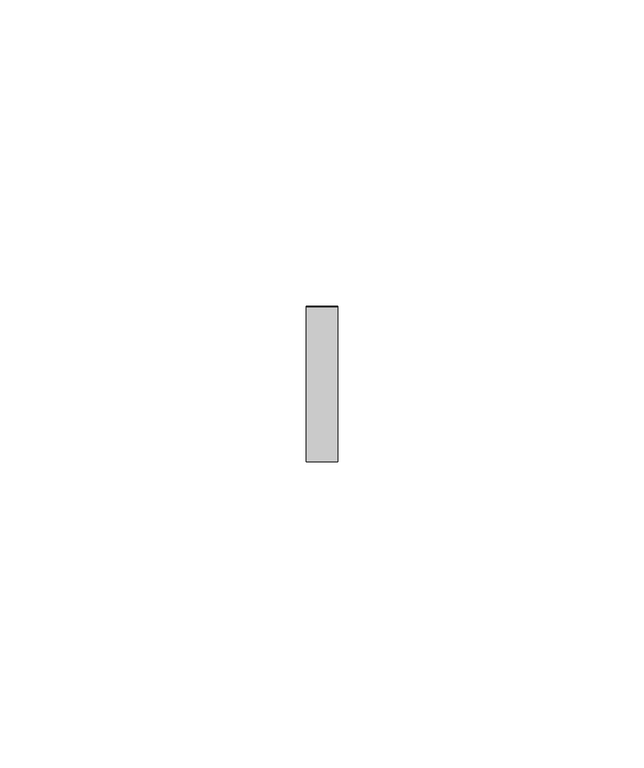
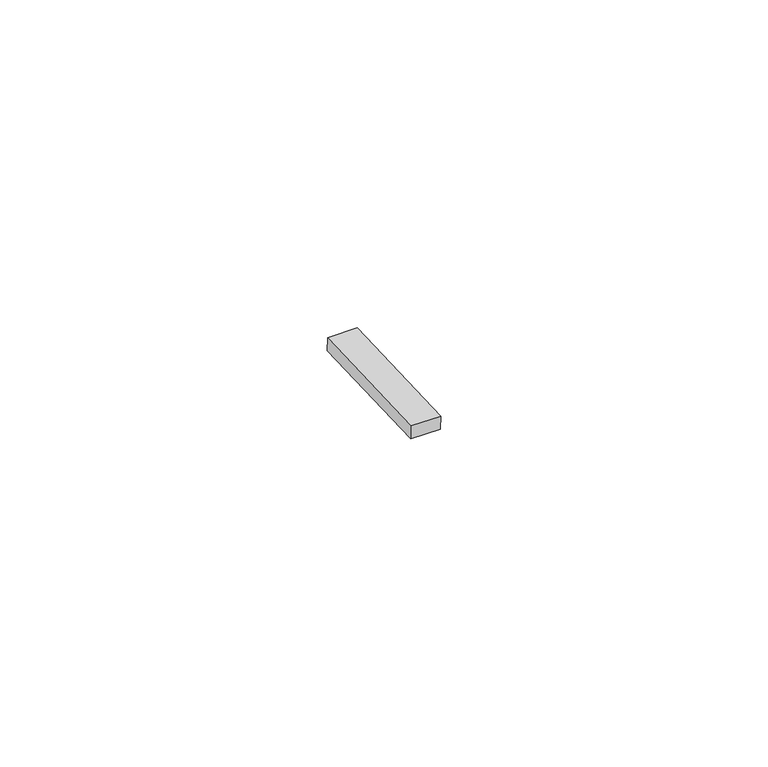
"""IFC4 building model written with IfcOpenShell, lengths in millimetres: proxy geometry, Inner panel:Inner panel:1:Inner panel:1 : Inner panel:Inner panel:300324:2:Inner panel:1:Inner panel:1 : Inner panel:Inner panel:300324:2 : Inner panel:Inner panel:1:Inner panel:1 : Inner panel:Inner panel:300324:300043:113 : Inner panel:Inner panel:1:Inner panel:1 : Inner panel:Inner panel:300324:2:Inner panel:1:Inner panel:1 : Inner panel:Inner panel:300324:2 : Inner panel:Inner panel:1:Inner panel:1 : Inner panel:Inner panel:300324:300043:308120."""

from ifc_helpers import new_model, si_unit, frame, origin, place, context, project, spatial, polyline, outline, extrude, source, transform, mapped, element, save


def generic_models_d7753da4(model_context):
    return source(origin(), model_context, "Body", "SweptSolid", [
        extrude(outline(polyline([(0.0, -25.4), (0.0, 0.0), (5.2138089, 0.0), (5.2138089, -25.4), (0.0, -25.4)])), frame((593936.595117, -578253.2828061, 3981.0403755), z_axis=(0.0, -0.041630544712223896, 0.9991330730923502), x_axis=(-1.0, 0.0, 0.0)), (0.0, 0.0, 1.0), 2.4763745),
    ])


if __name__ == "__main__":
    model = new_model("IFC4")
    model_context = context("Model", 3, world=origin())
    ifc_project = project(units=[si_unit("LENGTHUNIT", "METRE", prefix="MILLI")], contexts=[model_context])
    site = spatial("IfcSite", under=ifc_project)
    building = spatial("IfcBuilding", under=site)
    placement = place(None, origin())
    generic_models_shape = generic_models_d7753da4(model_context)
    element("IfcBuildingElementProxy", 1, Name="Inner panel:Inner panel:1:Inner panel:1 : Inner panel:Inner panel:300324:2:Inner panel:1:Inner panel:1 : Inner panel:Inner panel:300324:2 : Inner panel:Inner panel:1:Inner panel:1 : Inner panel:Inner panel:300324:300043:113 : Inner panel:Inner panel:1:Inner panel:1 : Inner panel:Inner panel:300324:2:Inner panel:1:Inner panel:1 : Inner panel:Inner panel:300324:2 : Inner panel:Inner panel:1:Inner panel:1 : Inner panel:Inner panel:300324:300043:308120", ObjectType="Inner panel:Inner panel:1:Inner panel:1 : Inner panel:Inner panel:300324:2:Inner panel:1:Inner panel:1 : Inner panel:Inner panel:300324:2 : Inner panel:Inner panel:1:Inner panel:1 : Inner panel:Inner panel:300324:300043:113 : Inner panel:Inner panel:1:Inner panel:1 : Inner panel:Inner panel:300324:2:Inner panel:1:Inner panel:1 : Inner panel:Inner panel:300324:2 : Inner panel:Inner panel:1:Inner panel:1 : Inner panel:Inner panel:300324:300043:308120", at=placement, inside=building, context=model_context, shape_type="MappedRepresentation", body=[
        mapped(generic_models_shape, transform((0.0, 0.0, 0.0), x_axis=(1.0, 0.0, 0.0), y_axis=(0.0, 1.0, 0.0), z_axis=(0.0, 0.0, 1.0))),
    ])
    save(model, "model.ifc")

# Revit data of these elements
# Type "Inner panel:Inner panel:1:Inner panel:1 : Inner panel:Inner panel:300324:2:Inner panel:1:Inner panel:1 : Inner panel:Inner panel:300324:2 : Inner panel:Inner panel:1:Inner panel:1 : Inner panel:Inner panel:300324:300043:113 : Inner panel:Inner panel:1:Inner panel:1 : Inner panel:Inner panel:300324:2:Inner panel:1:Inner panel:1 : Inner panel:Inner panel:300324:2 : Inner panel:Inner panel:1:Inner panel:1 : Inner panel:Inner panel:300324:300043:308120"
#   NameOverride = "Inner panel:Inner panel:1:Inner panel:1 : Inner panel:Inner panel:300324:2:Inner panel:1:Inner panel:1 : Inner panel:Inner panel:300324:2 : Inner panel:Inner panel:1:Inner panel:1 : Inner panel:Inner panel:300324:300043:308120"
#   ObjectTypeOverride = "Inner panel:1:Inner panel:1 : Inner panel:Inner panel:300324:2 : Inner panel:Inner panel:1:Inner panel:1 : Inner panel:Inner panel:300324:300043"
#   Reference = "Inner panel"
#   Tag = "308120"
# Element 1 (IfcBuildingElementProxy, "Inner panel:Inner panel:1:Inner panel:1 : Inner panel:Inner panel:300324:2:Inner panel:1:Inner panel:1 : Inner panel:Inner panel:300324:2 : Inner panel:Inner panel:1:Inner panel:1 : Inner panel:Inner panel:300324:300043:113 : Inner panel:Inner panel:1:Inner panel:1 : Inner panel:Inner panel:300324:2:Inner panel:1:Inner panel:1 : Inner panel:Inner panel:300324:2 : Inner panel:Inner panel:1:Inner panel:1 : Inner panel:Inner panel:300324:300043:308120")
#   Materials on its faces: "AT CLIP - 1\" WIDE NON ABSORBENT, WEATHER-RESISTANT NEOPRENE/EPDM/SBR FOAM"
# Materials
#   "AT CLIP - 1\" WIDE NON ABSORBENT, WEATHER-RESISTANT NEOPRENE/EPDM/SBR FOAM": class "Generic", colour RGB 85 85 85, transparency 0, Cost = 0
